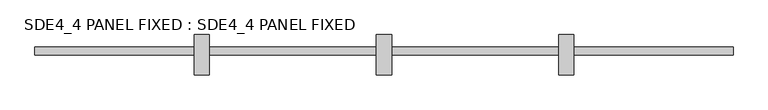
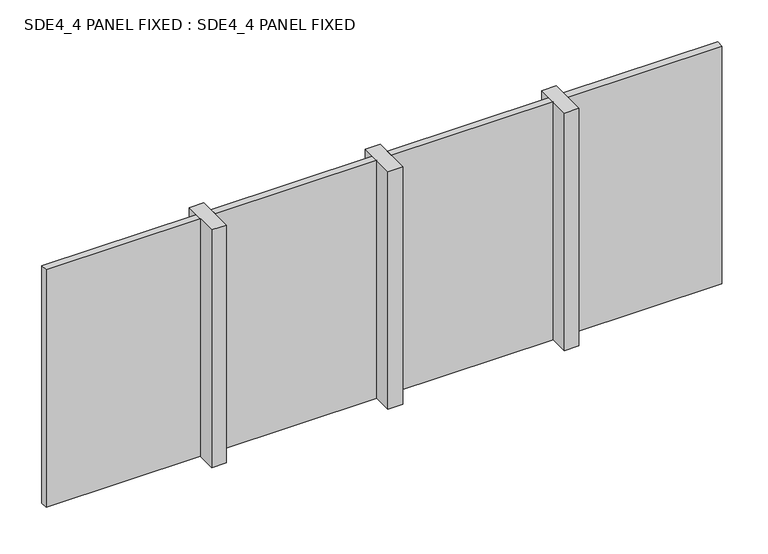
"""IFC4 building model written with IfcOpenShell, lengths in millimetres: plate geometry, SDE4_4 PANEL FIXED : SDE4_4 PANEL FIXED."""

from ifc_helpers import new_model, si_unit, origin, origin_with_axes, place, context, project, spatial, polyline, outline, extrude, source, transform, mapped, element, save


def sde4_4_panel_fixed_sde4_4_panel_fixed_757810fe(model_context):
    return source(origin(), model_context, "Body", "SweptSolid", [
        extrude(outline(polyline([(-1150.0, 132.5), (-1150.0, -132.5), (-1250.0, -132.5), (-1250.0, 132.5), (-1150.0, 132.5)])), origin_with_axes(), (0.0, 0.0, 1.0), 1710.0),
        extrude(outline(polyline([(50.0, 132.5), (50.0, -132.5), (-50.0, -132.5), (-50.0, 132.5), (50.0, 132.5)])), origin_with_axes(), (0.0, 0.0, 1.0), 1710.0),
        extrude(outline(polyline([(1250.0, 132.5), (1250.0, -132.5), (1150.0, -132.5), (1150.0, 132.5), (1250.0, 132.5)])), origin_with_axes(), (0.0, 0.0, 1.0), 1710.0),
        extrude(outline(polyline([(2299.0, 50.0), (2299.0, 0.0), (1250.0, 0.0), (1250.0, 50.0), (2299.0, 50.0)])), origin_with_axes(), (0.0, 0.0, 1.0), 1710.0),
        extrude(outline(polyline([(1150.0, 50.0), (1150.0, 0.0), (50.0, 0.0), (50.0, 50.0), (1150.0, 50.0)])), origin_with_axes(), (0.0, 0.0, 1.0), 1710.0),
        extrude(outline(polyline([(-50.0, 50.0), (-50.0, 0.0), (-1150.0, 0.0), (-1150.0, 50.0), (-50.0, 50.0)])), origin_with_axes(), (0.0, 0.0, 1.0), 1710.0),
        extrude(outline(polyline([(-1250.0, 50.0), (-1250.0, 0.0), (-2300.0, 0.0), (-2300.0, 50.0), (-1250.0, 50.0)])), origin_with_axes(), (0.0, 0.0, 1.0), 1710.0),
    ])


if __name__ == "__main__":
    model = new_model("IFC4")
    model_context = context("Model", 3, world=origin())
    ifc_project = project(units=[si_unit("LENGTHUNIT", "METRE", prefix="MILLI")], contexts=[model_context])
    site = spatial("IfcSite", under=ifc_project)
    building = spatial("IfcBuilding", under=site)
    placement = place(None, origin())
    sde4_4_panel_fixed_sde4_4_panel_fixed_shape = sde4_4_panel_fixed_sde4_4_panel_fixed_757810fe(model_context)
    element("IfcPlate", 1, ObjectType="SDE4_4 PANEL FIXED : SDE4_4 PANEL FIXED", at=placement, inside=building, context=model_context, shape_type="MappedRepresentation", body=[
        mapped(sde4_4_panel_fixed_sde4_4_panel_fixed_shape, transform((0.0, 0.0, 0.0), x_axis=(1.0, 0.0, 0.0), y_axis=(0.0, 1.0, 0.0), z_axis=(0.0, 0.0, 1.0))),
    ])
    save(model, "model.ifc")

# Revit data of these elements
# Type "SDE4_4 PANEL FIXED : SDE4_4 PANEL FIXED"
#   Type Mark = "CW-GLASS"
#   Analytic Construction = "<None>"
#   Glass = Glass
#   Frame = Aluminium
# Element 1 (IfcPlate, "SDE4_4 PANEL FIXED : SDE4_4 PANEL FIXED")
#   Materials on its faces: "Glass", "Aluminium"
# Materials
#   "Glass": class "Glass", colour RGB 0 128 192, transparency 0.9, Keynote = "L40", Cost = 0
#   "Aluminium": class "Unassigned", colour RGB 247 247 247, transparency 0, Cost = 0
